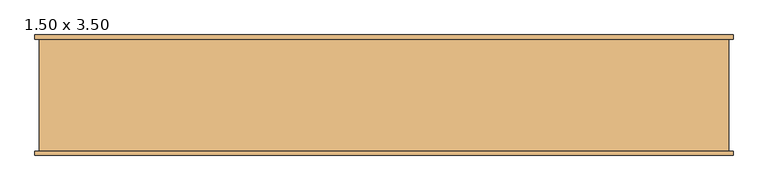
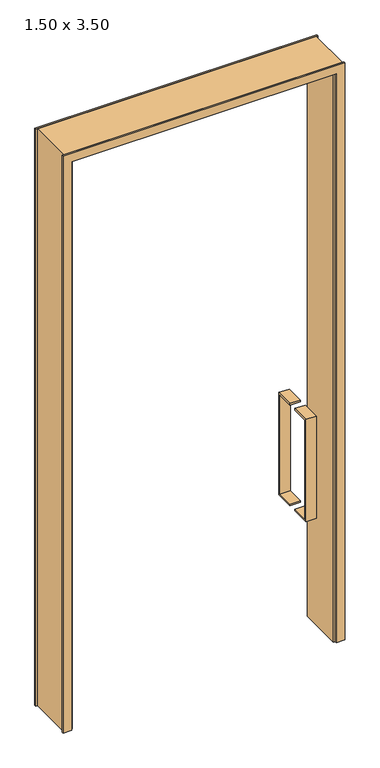
"""IFC4 building model written with IfcOpenShell, lengths in millimetres: door geometry, .CC_ND 300 PORTA PIVOTANTE_COM BANDEIRA_COM EXTENSÃO : 1.50 x 3.50."""

from ifc_helpers import new_model, si_unit, frame, origin, place, context, project, spatial, polyline, outline, extrude, source, transform, mapped, element, save


def door_1_50_x_3_50_a1620f17(model_context):
    return source(origin(), model_context, "Body", "SweptSolid", [
        extrude(outline(polyline([(0.0, -810.0), (0.0, -760.0), (3450.0, -760.0), (3450.0, 760.0), (0.0, 760.0), (0.0, 810.0), (3500.0, 810.0), (3500.0, -810.0), (0.0, -810.0)])), frame((0.0, -139.9, 0.0), z_axis=(0.0, 1.0, 0.0), x_axis=(0.0, 0.0, 1.0)), (0.0, 0.0, 1.0), 10.0),
        extrude(outline(polyline([(0.0, 760.0), (0.0, 810.0), (3500.0, 810.0), (3500.0, -810.0), (0.0, -810.0), (0.0, -760.0), (3450.0, -760.0), (3450.0, 760.0), (0.0, 760.0)])), frame((0.0, 129.9, 0.0), z_axis=(0.0, 1.0, 0.0), x_axis=(0.0, 0.0, 1.0)), (0.0, 0.0, 1.0), 10.0),
        extrude(outline(polyline([(0.0, -800.0), (0.0, -750.0), (3450.0, -750.0), (3450.0, 750.0), (0.0, 750.0), (0.0, 800.0), (3500.0, 800.0), (3500.0, -800.0), (0.0, -800.0)])), frame((0.0, -129.9, 0.0), z_axis=(0.0, 1.0, 0.0), x_axis=(0.0, 0.0, 1.0)), (0.0, 0.0, 1.0), 259.8),
        extrude(outline(polyline([(-25.0, 1410.0), (-25.0, 1400.0), (-125.0, 1400.0), (-125.0, 800.0), (-25.0, 800.0), (-25.0, 790.0), (-135.0, 790.0), (-135.0, 1410.0), (-25.0, 1410.0)])), frame((590.0, 0.0, 0.0), z_axis=(1.0, 0.0, 0.0), x_axis=(0.0, 1.0, 0.0)), (0.0, 0.0, 1.0), 60.0),
        extrude(outline(polyline([(25.0, 1400.0), (25.0, 1410.0), (135.0, 1410.0), (135.0, 790.0), (25.0, 790.0), (25.0, 800.0), (125.0, 800.0), (125.0, 1400.0), (25.0, 1400.0)])), frame((590.0, 0.0, 0.0), z_axis=(1.0, 0.0, 0.0), x_axis=(0.0, 1.0, 0.0)), (0.0, 0.0, 1.0), 60.0),
    ])


if __name__ == "__main__":
    model = new_model("IFC4")
    model_context = context("Model", 3, world=origin())
    ifc_project = project(units=[si_unit("LENGTHUNIT", "METRE", prefix="MILLI")], contexts=[model_context])
    site = spatial("IfcSite", under=ifc_project)
    building = spatial("IfcBuilding", under=site)
    placement = place(None, origin())
    door_1_50_x_3_50_shape = door_1_50_x_3_50_a1620f17(model_context)
    element("IfcDoor", 1, ObjectType=".CC_ND 300 PORTA PIVOTANTE_COM BANDEIRA_COM EXTENSÃO : 1.50 x 3.50", at=placement, inside=building, context=model_context, shape_type="MappedRepresentation", body=[
        mapped(door_1_50_x_3_50_shape, transform((0.0, 0.0, 0.0), x_axis=(1.0, 0.0, 0.0), y_axis=(0.0, 1.0, 0.0), z_axis=(0.0, 0.0, 1.0))),
    ])
    save(model, "model.ifc")

# Revit data of these elements
# Type ".CC_ND 300 PORTA PIVOTANTE_COM BANDEIRA_COM EXTENSÃO : 1.50 x 3.50"
#   Type Mark = "151"
#   Pivot = 0.10 m
#   Largura moldura = 0.05 m
#   Rough Width = 1.60 m
#   Extensão do acabamento interior [instance default] = 0.00 m
#   Extensão do acabamento exterior [instance default] = 0.00 m
#   Espessura moldura = 0.01 m
#   Espessura batente = 0.05 m
#   Thickness = 0.05 m
#   Rough Height = 3.50 m
#   Altura bandeira = 1.35 m
#   Height = 2.10 m
#   Width = 1.50 m
#   Puxador interno [instance default] = yes
#   Puxador externo [instance default] = yes
#   Número de ripas da porta = 4
#   Moldura interna [instance default] = yes
#   Moldura externa [instance default] = yes
#   Function = 1
#   Puxador = .ALUMÍNIO
#   Porta = .MADEIRA_CEREJEIRA CLARO
#   Moldura = .MADEIRA_CEREJEIRA CLARO
#   Batente = .MADEIRA_CEREJEIRA CLARO
#   Wall Closure = (empty or 0)
# Element 1 (IfcDoor, ".CC_ND 300 PORTA PIVOTANTE_COM BANDEIRA_COM EXTENSÃO : 1.50 x 3.50")
#   Materials on its faces: ".MADEIRA_CEREJEIRA CLARO", ".ALUMÍNIO"
# Materials
#   ".ALUMÍNIO": class "CC_METAIS", colour RGB 244 244 244, transparency 0, Description = "Material alumínio", Cost = 0
#   ".MADEIRA_CEREJEIRA CLARO": class ".CC_MADEIRA REVEST.", colour RGB 233 182 144, transparency 0, Cost = 0
